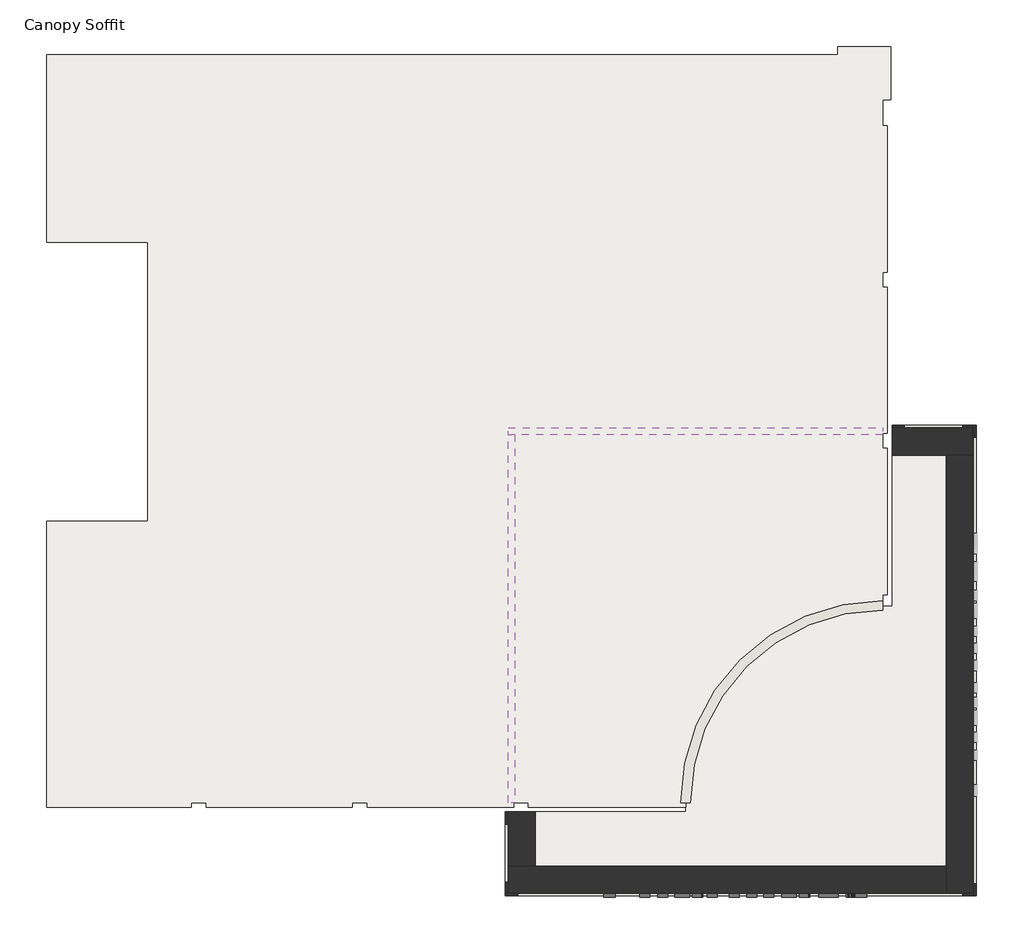
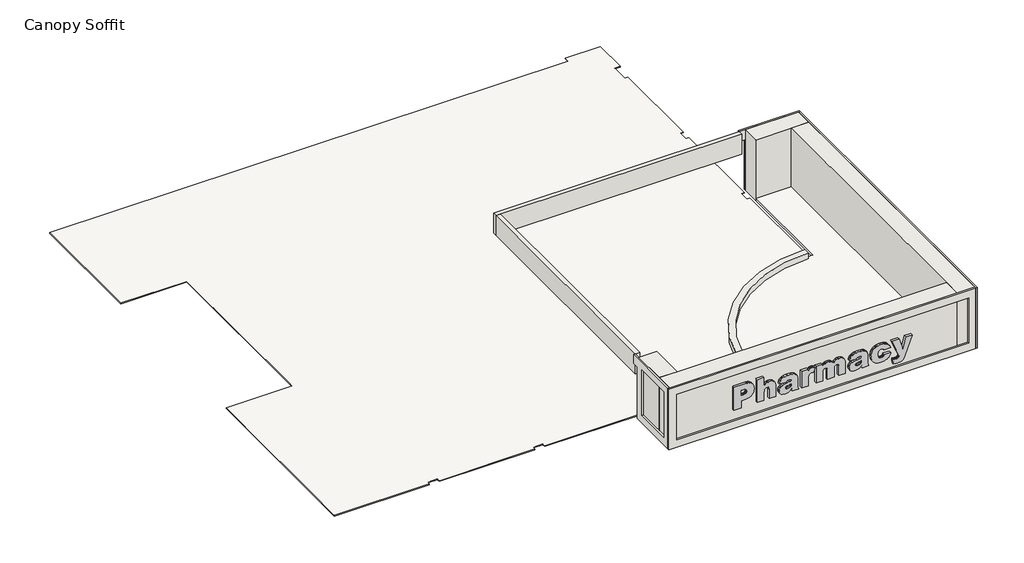
# One storey, part 1 of 2: 11 walls, 2 coverings, 1 proxy.
"""IFC4 building model written with IfcOpenShell, lengths in millimetres."""

from ifc_helpers import new_model, si_unit, point, frame, frame_2d, origin, place, context, project, spatial, polyline, circle_curve, trimmed, segment, composite_curve, outline, extrude, faceted_brep, element, save
from ifc_brep_helpers import plane_surface, cylinder_surface, revolved_surface, advanced_brep

model = new_model("IFC4")

# Units and contexts
model_context = context("Model", 3, world=origin())
ifc_project = project(units=[si_unit("LENGTHUNIT", "METRE", prefix="MILLI")], contexts=[model_context])

# Site, building, storey
site = spatial("IfcSite", under=ifc_project)
building = spatial("IfcBuilding", under=site)
storey = spatial("IfcBuildingStorey", under=building, Name="Canopy Soffit", Elevation=4572.0)

# Proxy
placement = place(None, origin())
element("IfcBuildingElementProxy", 1, Name="big", ObjectType="big", at=placement, inside=storey, context=model_context, shape_type="SweptSolid", body=[
    extrude(outline(polyline([(7079.97721, 8014.3522712), (5707.3420402, 8014.3522712), (5707.3420402, 8444.9829127), (6137.9726817, 8444.9829127), (6137.9726817, 8673.3349032), (6139.9669505, 8734.3950112), (6145.9497569, 8791.4140144), (6155.9211009, 8844.3919127), (6169.8809824, 8893.3287063), (6187.8294016, 8938.2243951), (6209.7663583, 8979.078979), (6235.6918526, 9015.8924581), (6265.6058845, 9048.6648325), (6299.0682036, 9077.4946655), (6335.6385594, 9102.4805209), (6375.3169518, 9123.6223984), (6418.103381, 9140.9202983), (6463.9978469, 9154.3742204), (6513.0003495, 9163.9841647), (6565.1108887, 9169.7501313), (6620.3294647, 9171.6721202), (6673.8461771, 9169.8914057), (6724.2154273, 9164.5492623), (6771.4372154, 9155.6456899), (6815.5115414, 9143.1806886), (6856.4384053, 9127.1542583), (6894.217807, 9107.5663991), (6928.8497466, 9084.4171109), (6960.3342242, 9057.7063938), (6988.375549, 9027.4211059), (7012.6780305, 8993.5481055), (7033.2416687, 8956.0873925), (7050.0664636, 8915.0389669), (7063.1524151, 8870.4028288), (7072.4995234, 8822.1789781), (7078.1077884, 8770.3674149), (7079.97721, 8714.9681391), (7079.97721, 8014.3522712)]), holes=[polyline([(6460.9456628, 8444.9829127), (6757.0042289, 8444.9829127), (6757.0042289, 8554.7432617), (6754.2838754, 8604.471849), (6746.122815, 8645.5794127), (6732.5210476, 8678.0659528), (6713.4785732, 8701.9314693), (6690.5461248, 8719.0420984), (6665.2744353, 8731.2639763), (6637.6635045, 8738.5971031), (6607.7133327, 8741.0414787), (6576.9877943, 8738.2291326), (6549.1534529, 8729.7920943), (6524.2103085, 8715.7303637), (6502.158361, 8696.043941), (6484.1278055, 8669.392362), (6471.2488374, 8634.4351627), (6463.5214565, 8591.1723431), (6460.9456628, 8539.6039032), (6460.9456628, 8444.9829127)])]), frame((0.0, -17607.3313057, 0.0), z_axis=(0.0, 1.0, 0.0), x_axis=(0.0, 0.0, 1.0)), (0.0, 0.0, 1.0), 152.4),
    extrude(outline(polyline([(7079.97721, 9360.0730259), (5707.3420402, 9360.0730259), (5707.3420402, 9736.8748372), (6190.5398987, 9736.8748372), (6254.0148132, 9739.6477579), (6306.9237171, 9747.96652), (6349.2666104, 9761.8311235), (6381.043493, 9781.2415683), (6404.2256357, 9805.1202266), (6420.7843091, 9832.3894704), (6430.7195131, 9863.0492998), (6434.0312478, 9897.0997146), (6431.5737304, 9927.483566), (6424.2011782, 9954.2928466), (6411.9135912, 9977.5275565), (6394.7109695, 9997.1876957), (6371.5945358, 10012.8264427), (6341.5655131, 10023.9969763), (6304.6239014, 10030.6992965), (6260.7697006, 10032.9334032), (5707.3420402, 10032.9334032), (5707.3420402, 10409.7352146), (6343.1950968, 10409.7352146), (6435.2402937, 10404.1236641), (6476.4924173, 10397.1092261), (6514.5642242, 10387.2890129), (6549.4557144, 10374.6630245), (6581.1668881, 10359.2312608), (6609.6977451, 10340.993722), (6635.0482855, 10319.9504079), (6657.3236437, 10296.4692892), (6676.6289541, 10270.9183363), (6692.9642168, 10243.2975492), (6706.3294317, 10213.606928), (6716.7245989, 10181.8464726), (6724.1497183, 10148.016183), (6730.0898138, 10074.1461013), (6727.9345579, 10023.3267443), (6721.4687902, 9976.0031072), (6710.6925107, 9932.1751901), (6695.6057195, 9891.8429929), (6675.498759, 9853.2192302), (6649.6619718, 9814.5166167), (6618.095358, 9775.7351523), (6580.7989176, 9736.8748372), (7079.97721, 9736.8748372), (7079.97721, 9360.0730259)])), frame((0.0, -17607.3313057, 0.0), z_axis=(0.0, 1.0, 0.0), x_axis=(0.0, 0.0, 1.0)), (0.0, 0.0, 1.0), 152.4),
    extrude(outline(polyline([(6353.2880025, 11001.8523466), (6380.3864028, 11012.7337605), (6402.8063209, 11025.192191), (6420.5477566, 11039.2276379), (6433.61071, 11054.8401013), (6445.5697519, 11078.3113637), (6454.1119246, 11107.091915), (6459.2372283, 11141.1817552), (6460.9456628, 11180.5808844), (6459.4474972, 11210.7281833), (6454.9530001, 11235.9867311), (6447.4621717, 11256.3565276), (6436.9750119, 11271.837573), (6422.7555797, 11283.2446591), (6404.0679341, 11291.3925778), (6380.912075, 11296.2813289), (6353.2880025, 11297.9109127), (6328.5288433, 11231.0979799), (6308.9212713, 11167.7544834), (6285.5288598, 11069.8217582), (6249.4151817, 10899.2411391), (6229.6761917, 10819.628089), (6205.3638539, 10753.629948), (6176.4781682, 10701.2467163), (6143.0191345, 10662.4783938), (6104.8027678, 10634.3286491), (6061.6450827, 10614.2216886), (6013.5460791, 10602.1575123), (5960.5057572, 10598.1361202), (5903.5754612, 10603.7082452), (5851.3762147, 10620.4246202), (5803.9080178, 10648.2852452), (5761.1708704, 10687.2901202), (5742.2466723, 10710.8730879), (5725.8457006, 10737.0449911), (5711.9679553, 10765.8058297), (5700.6134364, 10797.1556037), (5685.4740779, 10867.6219581), (5680.4276251, 10948.4440542), (5683.6867926, 11011.2355949), (5693.4642949, 11070.0845943), (5709.7601322, 11124.9910524), (5732.5743044, 11175.9549693), (5755.5724618, 11211.753244), (5785.0363869, 11247.6566532), (5820.9660797, 11283.6651969), (5863.3615402, 11319.7788749), (5782.4080261, 11333.0258136), (5707.3420402, 11361.4121108), (5707.3420402, 11722.6540259), (5764.0095001, 11697.737165), (5809.53271, 11683.5440164), (5857.1586086, 11676.9205471), (5920.1341345, 11674.712724), (6361.6987572, 11674.712724), (6397.4707483, 11672.9911476), (6434.1363822, 11667.8264186), (6510.1485779, 11647.1675023), (6546.8404954, 11632.1201364), (6579.1167666, 11614.5232605), (6606.9773916, 11594.3768746), (6630.4223704, 11571.6809787), (6658.309279, 11535.4884498), (6680.9920331, 11495.0379763), (6698.4706328, 11450.3295583), (6710.7450779, 11401.3631957), (6719.2083999, 11346.1150506), (6725.2536298, 11282.5612853), (6730.0898138, 11130.5368938), (6725.5164659, 11029.1347322), (6711.7964223, 10935.1971155), (6689.8758928, 10854.7167063), (6676.1952746, 10821.7702031), (6660.7010874, 10793.6861674), (6636.559593, 10759.8328796), (6610.3942607, 10730.1849693), (6582.2050906, 10704.7424363), (6551.9920827, 10683.5052806), (6517.8365334, 10665.5010088), (6477.8197395, 10649.7571273), (6431.9417009, 10636.2736361), (6380.2024176, 10625.0505353), (6353.2880025, 11001.8523466)]), holes=[polyline([(6164.8870968, 11297.9109127), (6118.6279459, 11297.9109127), (6069.477598, 11292.4964893), (6048.7266891, 11285.7284601), (6030.5252902, 11276.2532193), (6014.2425947, 11263.5582364), (5999.2477961, 11247.1309811), (5973.1218893, 11203.0796532), (5955.4593044, 11149.4085247), (5949.5717761, 11091.4268844), (5954.9861994, 11041.1200577), (5961.7542286, 11021.1313735), (5971.2294695, 11004.5858419), (5982.8599662, 10991.6148811), (5996.0937631, 10982.3499091), (6010.9308601, 10976.7909259), (6027.3712572, 10974.9379315), (6041.9060927, 10976.8040677), (6055.6524199, 10982.4024763), (6068.6102389, 10991.7331574), (6080.7795496, 11004.7961108), (6092.1866357, 11024.5088171), (6103.6988562, 11054.2092947), (6127.0387006, 11143.5735636), (6144.7012855, 11222.3192546), (6164.8870968, 11297.9109127)])]), frame((0.0, -17607.3313057, 0.0), z_axis=(0.0, 1.0, 0.0), x_axis=(0.0, 0.0, 1.0)), (0.0, 0.0, 1.0), 152.4),
    extrude(outline(polyline([(6703.1753987, 11890.0280447), (5707.3420402, 11890.0280447), (5707.3420402, 12266.8298561), (6043.3516912, 12266.8298561), (6154.0845337, 12270.5621285), (6245.7354765, 12281.7589457), (6318.3045196, 12300.4203077), (6347.4333287, 12312.550193), (6371.7916628, 12326.5462146), (6399.0214812, 12349.4918048), (6418.4713515, 12376.6953396), (6430.1412737, 12408.1568189), (6434.0312478, 12443.8762429), (6426.9872407, 12490.5559315), (6405.8552195, 12551.5339032), (6673.7377572, 12670.5460825), (6698.391782, 12621.0803313), (6716.0017996, 12573.6121344), (6726.5678103, 12528.1414917), (6730.0898138, 12484.6684032), (6727.5797292, 12445.7029536), (6720.0494753, 12409.9703879), (6707.4990523, 12377.470706), (6689.92846, 12348.2039079), (6665.6818312, 12320.7769625), (6633.1032985, 12293.7968384), (6592.1928618, 12267.2635356), (6542.9505213, 12241.1770542), (6703.1753987, 12241.1770542), (6703.1753987, 11890.0280447)])), frame((0.0, -17607.3313057, 0.0), z_axis=(0.0, 1.0, 0.0), x_axis=(0.0, 0.0, 1.0)), (0.0, 0.0, 1.0), 152.4),
    extrude(outline(polyline([(6703.1753987, 12724.3749127), (5707.3420402, 12724.3749127), (5707.3420402, 13101.176724), (6219.5570025, 13101.176724), (6272.7287424, 13103.8050848), (6317.8576982, 13111.6901674), (6354.9438698, 13124.8319716), (6383.9872572, 13143.2304976), (6405.8815031, 13165.7292664), (6421.5202501, 13191.1717995), (6430.9034983, 13219.5580966), (6434.0312478, 13250.8881579), (6428.2488539, 13288.3160164), (6410.9016723, 13320.6974221), (6384.0923916, 13346.1399551), (6349.9237006, 13362.7511957), (6315.7550095, 13368.4284551), (6260.3491628, 13370.3208749), (5707.3420402, 13370.3208749), (5707.3420402, 13747.1226863), (6226.706144, 13747.1226863), (6277.4335084, 13749.6721963), (6320.6963279, 13757.3207263), (6356.4946027, 13770.0682765), (6384.8283327, 13787.9148466), (6406.354608, 13809.9405105), (6421.730519, 13835.2253419), (6430.9560656, 13863.7693407), (6434.0312478, 13895.572507), (6430.7720803, 13922.7760418), (6420.9945779, 13947.6140518), (6404.6987407, 13970.0865371), (6381.8845685, 13990.1934976), (6363.0917884, 14001.6005837), (6339.9359294, 14009.7485023), (6312.4169913, 14014.6372535), (6280.5349742, 14016.2668372), (5707.3420402, 14016.2668372), (5707.3420402, 14393.0686485), (6335.6254176, 14393.0686485), (6430.4698188, 14387.5096653), (6472.8554229, 14380.5609363), (6511.8832961, 14370.8327157), (6547.5534383, 14358.3250035), (6579.8658495, 14343.0377998), (6608.8205297, 14324.9711044), (6634.4174789, 14304.1249174), (6656.8406824, 14280.8080712), (6676.2741254, 14255.3293982), (6692.717808, 14227.6888984), (6706.1717301, 14197.8865719), (6716.6358917, 14165.9224185), (6724.1102929, 14131.7964383), (6730.0898138, 14057.0589976), (6727.8951325, 14005.5694085), (6721.3110886, 13958.3377641), (6710.337682, 13915.3640642), (6694.9749128, 13876.6483089), (6673.5406301, 13839.0890324), (6644.3526829, 13799.5847688), (6607.4110712, 13758.1355182), (6562.7157949, 13714.7412806), (6601.7732371, 13691.3225854), (6635.6790921, 13664.8024245), (6664.4333598, 13635.1807977), (6688.0360402, 13602.4577051), (6706.4345662, 13565.1086975), (6719.5763704, 13521.6093254), (6727.4614529, 13471.959589), (6730.0898138, 13416.1594881), (6727.6980054, 13363.3031515), (6720.5225803, 13314.4944905), (6708.5635384, 13269.7335052), (6691.8208798, 13229.0201957), (6669.4009618, 13190.4095748), (6640.4101416, 13151.9566556), (6604.8484193, 13113.661438), (6562.7157949, 13075.5239221), (6703.1753987, 13075.5239221), (6703.1753987, 12724.3749127)])), frame((0.0, -17607.3313057, 0.0), z_axis=(0.0, 1.0, 0.0), x_axis=(0.0, 0.0, 1.0)), (0.0, 0.0, 1.0), 152.4),
    extrude(outline(polyline([(6353.2880025, 15012.1001957), (6380.3864028, 15022.9816096), (6402.8063209, 15035.44004), (6420.5477566, 15049.475487), (6433.61071, 15065.0879504), (6445.5697519, 15088.5592128), (6454.1119246, 15117.3397641), (6459.2372283, 15151.4296043), (6460.9456628, 15190.8287334), (6459.4474972, 15220.9760324), (6454.9530001, 15246.2345801), (6447.4621717, 15266.6043767), (6436.9750119, 15282.0854221), (6422.7555797, 15293.4925082), (6404.0679341, 15301.6404268), (6380.912075, 15306.529178), (6353.2880025, 15308.1587617), (6328.5288433, 15241.3458289), (6308.9212713, 15178.0023325), (6285.5288598, 15080.0696072), (6249.4151817, 14909.4889881), (6229.6761917, 14829.875938), (6205.3638539, 14763.8777971), (6176.4781682, 14711.4945654), (6143.0191345, 14672.7262429), (6104.8027678, 14644.5764982), (6061.6450827, 14624.4695377), (6013.5460791, 14612.4053614), (5960.5057572, 14608.3839693), (5903.5754612, 14613.9560943), (5851.3762147, 14630.6724693), (5803.9080178, 14658.5330943), (5761.1708704, 14697.5379693), (5742.2466723, 14721.120937), (5725.8457006, 14747.2928401), (5711.9679553, 14776.0536787), (5700.6134364, 14807.4034528), (5685.4740779, 14877.8698071), (5680.4276251, 14958.6919032), (5683.6867926, 15021.4834439), (5693.4642949, 15080.3324433), (5709.7601322, 15135.2389015), (5732.5743044, 15186.2028183), (5755.5724618, 15222.0010931), (5785.0363869, 15257.9045023), (5820.9660797, 15293.9130459), (5863.3615402, 15330.026724), (5782.4080261, 15343.2736627), (5707.3420402, 15371.6599598), (5707.3420402, 15732.9018749), (5764.0095001, 15707.9850141), (5809.53271, 15693.7918655), (5857.1586086, 15687.1683962), (5920.1341345, 15684.960573), (6361.6987572, 15684.960573), (6397.4707483, 15683.2389967), (6434.1363822, 15678.0742676), (6510.1485779, 15657.4153513), (6546.8404954, 15642.3679855), (6579.1167666, 15624.7711096), (6606.9773916, 15604.6247237), (6630.4223704, 15581.9288278), (6658.309279, 15545.7362989), (6680.9920331, 15505.2858254), (6698.4706328, 15460.5774074), (6710.7450779, 15411.6110447), (6719.2083999, 15356.3628997), (6725.2536298, 15292.8091344), (6730.0898138, 15140.7847429), (6725.5164659, 15039.3825813), (6711.7964223, 14945.4449646), (6689.8758928, 14864.9645554), (6676.1952746, 14832.0180521), (6660.7010874, 14803.9340164), (6636.559593, 14770.0807287), (6610.3942607, 14740.4328183), (6582.2050906, 14714.9902853), (6551.9920827, 14693.7531296), (6517.8365334, 14675.7488578), (6477.8197395, 14660.0049763), (6431.9417009, 14646.5214852), (6380.2024176, 14635.2983844), (6353.2880025, 15012.1001957)]), holes=[polyline([(6164.8870968, 15308.1587617), (6118.6279459, 15308.1587617), (6069.477598, 15302.7443384), (6048.7266891, 15295.9763092), (6030.5252902, 15286.5010683), (6014.2425947, 15273.8060854), (5999.2477961, 15257.3788301), (5973.1218893, 15213.3275023), (5955.4593044, 15159.6563738), (5949.5717761, 15101.6747334), (5954.9861994, 15051.3679068), (5961.7542286, 15031.3792225), (5971.2294695, 15014.833691), (5982.8599662, 15001.8627302), (5996.0937631, 14992.5977582), (6010.9308601, 14987.038775), (6027.3712572, 14985.1857806), (6041.9060927, 14987.0519168), (6055.6524199, 14992.6503254), (6068.6102389, 15001.9810064), (6080.7795496, 15015.0439598), (6092.1866357, 15034.7566662), (6103.6988562, 15064.4571438), (6127.0387006, 15153.8214127), (6144.7012855, 15232.5671037), (6164.8870968, 15308.1587617)])]), frame((0.0, -17607.3313057, 0.0), z_axis=(0.0, 1.0, 0.0), x_axis=(0.0, 0.0, 1.0)), (0.0, 0.0, 1.0), 152.4),
    extrude(outline(polyline([(6084.1438515, 16626.9651013), (6052.090991, 16613.9021479), (6024.4800603, 16597.8428631), (6001.3110594, 16578.787247), (5982.5839883, 16556.7352995), (5968.1411455, 16531.792155), (5957.8248291, 16504.062948), (5951.6350393, 16473.5476786), (5949.5717761, 16440.2463466), (5953.4617501, 16400.6500904), (5965.1316723, 16364.7072558), (5984.5815426, 16332.4178428), (6011.811361, 16303.7818513), (6046.5320078, 16280.3237308), (6088.4543633, 16263.5679304), (6137.5784276, 16253.5144501), (6193.9042006, 16250.16329), (6256.9191519, 16253.4224575), (6311.3919305, 16263.1999598), (6357.3225364, 16279.4957971), (6394.7109695, 16302.3099693), (6423.6886478, 16330.4071467), (6444.3869895, 16362.5519999), (6456.8059945, 16398.7445288), (6460.9456628, 16438.9847334), (6459.2503701, 16470.7090489), (6454.1644919, 16499.0164952), (6445.6880281, 16523.9070725), (6433.8209789, 16545.3807806), (6418.6159114, 16563.6216049), (6400.1253928, 16578.8135306), (6378.3494232, 16590.9565577), (6353.2880025, 16600.0506863), (6380.2024176, 16976.8524976), (6460.8405284, 16946.9811765), (6497.2958934, 16928.5662233), (6531.1754647, 16907.8317417), (6562.4792424, 16884.7777316), (6591.2072265, 16859.404193), (6617.359417, 16831.711126), (6640.9358138, 16801.6985306), (6661.8312825, 16768.7618837), (6679.9406888, 16732.2966624), (6695.2640325, 16692.3028666), (6707.8013138, 16648.7804964), (6717.5525325, 16601.7295517), (6724.5176888, 16551.1500327), (6730.0898138, 16439.4052712), (6727.1986169, 16358.1100701), (6718.5250261, 16284.5422499), (6704.0690414, 16218.7018107), (6683.8306628, 16160.5887523), (6667.2062805, 16126.5383375), (6646.7707749, 16092.934744), (6622.524146, 16059.7779719), (6594.466394, 16027.0680212), (6563.517445, 15996.3030574), (6530.5972253, 15968.9812464), (6495.7057351, 15945.1025881), (6458.8429742, 15924.6670825), (6404.0942177, 15902.2208808), (6342.8796935, 15886.1878796), (6275.1994016, 15876.5680789), (6201.0533421, 15873.3614787), (6130.4949951, 15876.0029814), (6067.2697749, 15883.9274893), (6011.3776814, 15897.1350026), (5962.8187147, 15915.6255212), (5919.3850517, 15938.7813802), (5878.8688692, 15965.984915), (5841.2701673, 15997.2361255), (5806.5889459, 16032.5350117), (5775.6531387, 16071.658163), (5749.2906794, 16114.3821686), (5727.5015679, 16160.7070285), (5710.2858044, 16210.6327429), (5697.2228509, 16265.6180518), (5687.8921699, 16327.1216957), (5682.2937613, 16395.1436745), (5680.4276251, 16469.6839881), (5683.3451057, 16546.6818192), (5692.0975473, 16616.6093596), (5706.68495, 16679.4666093), (5727.1073138, 16735.2535683), (5752.7863993, 16785.1792827), (5783.1439671, 16830.4527983), (5818.1800172, 16871.0741152), (5857.8945496, 16907.0432334), (5901.8933103, 16938.3207275), (5949.7820449, 16964.8671721), (6001.5607537, 16986.6825671), (6057.2294364, 17003.7669127), (6084.1438515, 16626.9651013)])), frame((0.0, -17607.3313057, 0.0), z_axis=(0.0, 1.0, 0.0), x_axis=(0.0, 0.0, 1.0)), (0.0, 0.0, 1.0), 152.4),
    extrude(outline(polyline([(6703.1753987, 17057.5957429), (5698.5107478, 17473.9281013), (5665.8796478, 17458.6310412), (5638.6366876, 17441.7569646), (5616.7818672, 17423.3058714), (5600.3151864, 17403.2777617), (5588.2641519, 17380.8578437), (5579.6562702, 17355.2313254), (5574.4915411, 17326.3982069), (5572.7699647, 17294.3584881), (5574.3206976, 17245.2344239), (5578.9728963, 17198.3707499), (5586.7265608, 17153.7674663), (5597.5816912, 17111.424573), (5326.7553893, 17141.2827523), (5309.4082077, 17289.8377075), (5303.6258138, 17394.0259315), (5309.1979388, 17488.3052352), (5316.163095, 17530.615274), (5325.9143138, 17569.7055707), (5338.451595, 17605.5761254), (5353.7749388, 17638.226938), (5371.884345, 17667.6580086), (5392.7798138, 17693.8693372), (5431.837256, 17728.589984), (5485.5083845, 17762.9426603), (5553.7931994, 17796.9273661), (5636.6917006, 17830.5441013), (6703.1753987, 18214.9155919), (6703.1753987, 17844.4218466), (6040.407927, 17663.1700825), (6703.1753987, 17463.8351957), (6703.1753987, 17057.5957429)])), frame((0.0, -17607.3313057, 0.0), z_axis=(0.0, 1.0, 0.0), x_axis=(0.0, 0.0, 1.0)), (0.0, 0.0, 1.0), 152.4),
])

# Coverings
element("IfcCovering", 2, ObjectType="24\" x 24\" ACT.", at=placement, inside=storey, context=model_context, shape_type="SweptSolid", body=[
    extrude(outline(composite_curve([segment(polyline([(18477.7022279, 12310.6936943), (18477.7022279, 11321.6811943), (18653.9147279, 11321.6811943), (18653.9147279, 5835.2811943), (18477.7022279, 5835.2811943), (18477.7022279, 5276.4811943), (18653.9147279, 5276.4811943), (18653.9147279, -209.9188057), (18477.7022279, -209.9188057), (18477.7022279, -768.7188057), (18653.9147279, -768.7188057), (18653.9147279, -6255.1188057), (18477.7022279, -6255.1188057), (18477.7022279, -6661.5188057)]), True, "CONTINUOUS"), segment(trimmed(circle_curve(frame_2d((18477.7022279, -14054.5063057)), 7392.9875), [point((18477.7022279, -6661.5188057))], [point((11086.8150464, -14230.7188057))], True, "CARTESIAN"), True, "CONTINUOUS"), segment(polyline([(11086.8150464, -14230.7188057), (5191.9147279, -14230.7188057), (5191.9147279, -14054.5063057), (4633.1147279, -14054.5063057), (4633.1147279, -14230.7188057), (-853.2852721, -14230.7188057), (-853.2852721, -14054.5063057), (-1412.0852721, -14054.5063057), (-1412.0852721, -14230.7188057), (-6898.4852721, -14230.7188057), (-6898.4852721, -14054.5063057), (-7457.2852721, -14054.5063057), (-7457.2852721, -14230.7188057), (-12883.3602721, -14230.7188057), (-12883.3602721, -3500.0125557), (-9095.5852721, -3500.0125557), (-9095.5852721, 6956.8499443), (-12883.3602721, 6956.8499443), (-12883.3602721, 13993.4436943), (16794.9522279, 13993.4436943), (16794.9522279, 14298.2436943), (18782.5022279, 14298.2436943), (18782.5022279, 12310.6936943), (18477.7022279, 12310.6936943)]), True, "CONTINUOUS")], self_intersect=False)), frame((0.0, 0.0, 4572.0), z_axis=(0.0, 0.0, 1.0), x_axis=(1.0, 0.0, 0.0)), (0.0, 0.0, 1.0), 38.1),
])
element("IfcCovering", 3, ObjectType="GWB on Mtl. Stud", at=placement, inside=storey, context=model_context, shape_type="SweptSolid", body=[
    extrude(outline(composite_curve([segment(polyline([(5445.9147279, -14406.9313057), (11093.1195861, -14406.9313057)]), True, "CONTINUOUS"), segment(trimmed(circle_curve(frame_2d((18477.7022279, -14054.5063057)), 7392.9875), [point((11093.1195861, -14406.9313057))], [point((18830.1272279, -6669.9236638))], False, "CARTESIAN"), True, "CONTINUOUS"), segment(polyline([(18830.1272279, -6669.9236638), (18830.1272279, -1022.7188057), (20862.1272279, -1022.7188057), (20862.1272279, -16438.9313057), (5445.9147279, -16438.9313057), (5445.9147279, -14406.9313057)]), True, "CONTINUOUS")], self_intersect=False)), frame((0.0, 0.0, 4572.0), z_axis=(0.0, 0.0, 1.0), x_axis=(1.0, 0.0, 0.0)), (0.0, 0.0, 1.0), 107.95),
])

# Walls
element("IfcWall", 4, ObjectType="Exterior - Brick on Mtl. Stud - No Cap", at=placement, inside=storey, context=model_context, shape_type="AdvancedBrep", body=[
    advanced_brep(
    [(18477.7022279, -6485.3063057, 5029.2), (10908.5022279, -14054.5063057, 5029.2), (11260.9272279, -14054.5063057, 5029.2), (18477.7022279, -6837.7313057, 5029.2), (10908.5022279, -14054.5063057, 3048.0), (18477.7022279, -6485.3063057, 3048.0), (18477.7022279, -6837.7313057, 3048.0), (18477.7022279, -6837.7313057, 4625.5040439), (11260.9272279, -14054.5063057, 4625.5040439), (11260.9272279, -14054.5063057, 3048.0)],
    [
        (0, 1, circle_curve(frame((18477.7022279, -14054.5063057, 5029.2), z_axis=(0.0, 0.0, 1.0), x_axis=(1.0, 0.0, 0.0)), 7569.2)),
        (1, 2),
        (2, 3, circle_curve(frame((18477.7022279, -14054.5063057, 5029.2), z_axis=(0.0, 0.0, -1.0), x_axis=(1.0, 0.0, 0.0)), 7216.775)),
        (3, 0),
        (4, 1),
        (0, 5),
        (5, 4, circle_curve(frame((18477.7022279, -14054.5063057, 3048.0), z_axis=(0.0, 0.0, 1.0), x_axis=(1.0, 0.0, 0.0)), 7569.2)),
        (6, 7),
        (7, 3),
        (2, 8),
        (8, 9),
        (9, 6, circle_curve(frame((18477.7022279, -14054.5063057, 3048.0), z_axis=(0.0, 0.0, -1.0), x_axis=(1.0, 0.0, 0.0)), 7216.775)),
        (6, 5),
        (4, 9),
    ],
    [
        plane_surface(frame((26046.9022279, -14054.5063057, 5029.2), z_axis=(0.0, 0.0, 1.0), x_axis=(0.0, 1.0, 0.0))),
        cylinder_surface(frame((18477.7022279, -14054.5063057, 4572.0), z_axis=(0.0, 0.0, 1.0), x_axis=(1.0, 0.0, 0.0)), 7569.2),
        revolved_surface(polyline([(25694.477227900003, -14054.5063057, 3048.0), (25694.477227900003, -14054.5063057, 5029.2)]), (18477.7022279, -14054.5063057, 4572.0), (0.0, 0.0, -1.0)),
        plane_surface(frame((18477.7022279, 12134.4811943, 7620.0), z_axis=(1.0, 0.0, 0.0), x_axis=(0.0, 0.0, -1.0))),
        plane_surface(frame((-12953.2102721, -14054.5063057, 7620.0), z_axis=(0.0, -1.0, 0.0), x_axis=(1.0, 0.0, 0.0))),
        plane_surface(frame((25883.3897279, -14054.5063057, 3048.0), z_axis=(0.0, 0.0, -1.0), x_axis=(0.0, 1.0, 0.0))),
    ],
    [
        (0, [[1, 2, 3, 4]]),
        (1, [[5, -1, 6, 7]]),
        (2, [[8, 9, -3, 10, 11, 12]]),
        (3, [[-4, -9, -8, 13, -6]]),
        (4, [[-2, -5, 14, -11, -10]]),
        (5, [[-13, -12, -14, -7]]),
    ],
),
])
element("IfcWall", 5, ObjectType="Exterior - EIFS Canopy Roof Wall", at=placement, inside=storey, context=model_context, shape_type="Brep", body=[
    faceted_brep([(18477.7022279, -6.7188057, 7016.75), (4429.9147279, -6.7188057, 7016.75), (4429.9147279, -6.7188057, 8229.6), (18477.7022279, -6.7188057, 8229.6), (18477.7022279, -254.3688057, 7016.75), (18477.7022279, -254.3688057, 8229.6), (4677.5647279, -254.3688057, 8229.6), (4429.9147279, -254.3688057, 8229.6), (4429.9147279, -254.3688057, 7016.75), (4677.5647279, -254.3688057, 7016.75)], [[[0, 1, 2, 3]], [[4, 5, 6, 7, 8, 9]], [[3, 2, 7, 6, 5]], [[0, 3, 5, 4]], [[2, 1, 8, 7]], [[1, 0, 4, 9, 8]]]),
])
element("IfcWall", 6, ObjectType="Exterior - EIFS Canopy Roof Wall", at=placement, inside=storey, context=model_context, shape_type="SweptSolid", body=[
    extrude(outline(polyline([(4677.5647279, -254.3688057), (4677.5647279, -14054.5063057), (4429.9147279, -14054.5063057), (4429.9147279, -254.3688057), (4677.5647279, -254.3688057)])), frame((0.0, 0.0, 7016.75), z_axis=(0.0, 0.0, 1.0), x_axis=(1.0, 0.0, 0.0)), (0.0, 0.0, 1.0), 1212.85),
])
element("IfcWall", 7, ObjectType="Exterior - EIFS Canopy Wall", at=placement, inside=storey, context=model_context, shape_type="Brep", body=[
    faceted_brep([(18830.1272279, -1022.7188057, 4572.0), (20862.1272279, -1022.7188057, 4572.0), (21878.1272279, -1022.7188057, 4572.0), (21878.1272279, -1022.7188057, 8229.6), (20862.1272279, -1022.7188057, 8229.6), (18830.1272279, -1022.7188057, 8229.6), (18830.1272279, -6.7188057, 4572.0), (18830.1272279, -6.7188057, 7620.0), (18830.1272279, -6.7188057, 8229.6), (21878.1272279, -6.7188057, 8229.6), (21878.1272279, -6.7188057, 4572.0)], [[[0, 1, 2, 3, 4, 5]], [[6, 7, 8, 9, 10]], [[2, 1, 0, 6, 10]], [[5, 4, 3, 9, 8]], [[0, 5, 8, 7, 6]], [[3, 2, 10, 9]]]),
])
element("IfcWall", 8, ObjectType="Exterior - EIFS Canopy Wall", at=placement, inside=storey, context=model_context, shape_type="Brep", body=[
    faceted_brep([(20862.1272279, -1022.7188057, 4572.0), (20862.1272279, -16438.9313057, 4572.0), (20862.1272279, -17454.9313057, 4572.0), (20862.1272279, -17454.9313057, 8229.6), (20862.1272279, -16438.9313057, 8229.6), (20862.1272279, -1022.7188057, 8229.6), (21878.1272279, -1022.7188057, 4572.0), (21878.1272279, -1022.7188057, 8229.6), (21878.1272279, -17454.9313057, 8229.6), (21878.1272279, -17454.9313057, 4572.0)], [[[0, 1, 2, 3, 4, 5]], [[6, 7, 8, 9]], [[2, 1, 0, 6, 9]], [[5, 4, 3, 8, 7]], [[0, 5, 7, 6]], [[3, 2, 9, 8]]]),
])
element("IfcWall", 9, ObjectType="Exterior - EIFS Canopy Wall", at=placement, inside=storey, context=model_context, shape_type="Brep", body=[
    faceted_brep([(20862.1272279, -16438.9313057, 4572.0), (5445.9147279, -16438.9313057, 4572.0), (4429.9147279, -16438.9313057, 4572.0), (4429.9147279, -16438.9313057, 8229.6), (5445.9147279, -16438.9313057, 8229.6), (20862.1272279, -16438.9313057, 8229.6), (20862.1272279, -17454.9313057, 4572.0), (20862.1272279, -17454.9313057, 8229.6), (4429.9147279, -17454.9313057, 8229.6), (4429.9147279, -17454.9313057, 4572.0)], [[[0, 1, 2, 3, 4, 5]], [[6, 7, 8, 9]], [[2, 1, 0, 6, 9]], [[5, 4, 3, 8, 7]], [[0, 5, 7, 6]], [[3, 2, 9, 8]]]),
])
element("IfcWall", 10, ObjectType="Exterior - EIFS Canopy Wall", at=placement, inside=storey, context=model_context, shape_type="Brep", body=[
    faceted_brep([(5445.9147279, -16438.9313057, 4572.0), (5445.9147279, -14406.9313057, 4572.0), (5445.9147279, -14406.9313057, 8229.6), (5445.9147279, -16438.9313057, 8229.6), (4429.9147279, -16438.9313057, 4572.0), (4429.9147279, -16438.9313057, 8229.6), (4429.9147279, -14406.9313057, 8229.6), (4429.9147279, -14406.9313057, 7683.5), (4429.9147279, -14406.9313057, 4572.0)], [[[0, 1, 2, 3]], [[4, 5, 6, 7, 8]], [[1, 0, 4, 8]], [[2, 1, 8, 7, 6]], [[3, 2, 6, 5]], [[0, 3, 5, 4]]]),
])
element("IfcWall", 11, ObjectType="Exterior - EIFS Details", at=placement, inside=storey, context=model_context, shape_type="Brep", body=[
    faceted_brep([(18830.1272279, -6.7188057, 4572.0), (21878.1272279, -6.7188057, 4572.0), (21979.7272279, -6.7188057, 4572.0), (21979.7272279, -6.7188057, 8229.6), (21878.1272279, -6.7188057, 8229.6), (18830.1272279, -6.7188057, 8229.6), (18477.7022279, -6.7188057, 8229.6), (18477.7022279, -6.7188057, 7620.0), (18830.1272279, -6.7188057, 7620.0), (21471.7272279, -6.7188057, 5029.2), (19287.3272279, -6.7188057, 5029.2), (19287.3272279, -6.7188057, 7772.4), (21471.7272279, -6.7188057, 7772.4), (18830.1272279, 94.8811943, 4572.0), (18830.1272279, 94.8811943, 7620.0), (18477.7022279, 94.8811943, 7620.0), (18477.7022279, 94.8811943, 8229.6), (21979.7272279, 94.8811943, 8229.6), (21979.7272279, 94.8811943, 4572.0), (21471.7272279, 94.8811943, 5029.2), (21471.7272279, 94.8811943, 7772.4), (19287.3272279, 94.8811943, 7772.4), (19287.3272279, 94.8811943, 5029.2)], [[[0, 1, 2, 3, 4, 5, 6, 7, 8], [9, 10, 11, 12]], [[13, 14, 15, 16, 17, 18], [19, 20, 21, 22]], [[3, 2, 18, 17]], [[2, 1, 0, 13, 18]], [[6, 5, 4, 3, 17, 16]], [[0, 8, 14, 13]], [[10, 9, 19, 22]], [[11, 10, 22, 21]], [[12, 11, 21, 20]], [[9, 12, 20, 19]], [[7, 6, 16, 15]], [[8, 7, 15, 14]]]),
])
element("IfcWall", 12, ObjectType="Exterior - EIFS Details", at=placement, inside=storey, context=model_context, shape_type="Brep", body=[
    faceted_brep([(21878.1272279, -6.7188057, 4572.0), (21878.1272279, -1022.7188057, 4572.0), (21878.1272279, -17454.9313057, 4572.0), (21878.1272279, -17556.5313057, 4572.0), (21878.1272279, -17556.5313057, 8229.6), (21878.1272279, -17454.9313057, 8229.6), (21878.1272279, -1022.7188057, 8229.6), (21878.1272279, -6.7188057, 8229.6), (21878.1272279, -362.3188057, 5029.2), (21878.1272279, -362.3188057, 7772.4), (21878.1272279, -17099.3313057, 7772.4), (21878.1272279, -17099.3313057, 5029.2), (21979.7272279, -6.7188057, 4572.0), (21979.7272279, -6.7188057, 8229.6), (21979.7272279, -17556.5313057, 8229.6), (21979.7272279, -17556.5313057, 4572.0), (21979.7272279, -362.3188057, 5029.2), (21979.7272279, -17099.3313057, 5029.2), (21979.7272279, -17099.3313057, 7772.4), (21979.7272279, -362.3188057, 7772.4)], [[[0, 1, 2, 3, 4, 5, 6, 7], [8, 9, 10, 11]], [[12, 13, 14, 15], [16, 17, 18, 19]], [[0, 7, 13, 12]], [[4, 3, 15, 14]], [[3, 2, 1, 0, 12, 15]], [[7, 6, 5, 4, 14, 13]], [[9, 8, 16, 19]], [[10, 9, 19, 18]], [[11, 10, 18, 17]], [[8, 11, 17, 16]]]),
])
element("IfcWall", 13, ObjectType="Exterior - EIFS Details", at=placement, inside=storey, context=model_context, shape_type="Brep", body=[
    faceted_brep([(21878.1272279, -17454.9313057, 4572.0), (20862.1272279, -17454.9313057, 4572.0), (4429.9147279, -17454.9313057, 4572.0), (4328.3147279, -17454.9313057, 4572.0), (4328.3147279, -17454.9313057, 8229.6), (4429.9147279, -17454.9313057, 8229.6), (20862.1272279, -17454.9313057, 8229.6), (21878.1272279, -17454.9313057, 8229.6), (4785.5147279, -17454.9313057, 5029.2), (21471.7272279, -17454.9313057, 5029.2), (21471.7272279, -17454.9313057, 7772.4), (4785.5147279, -17454.9313057, 7772.4), (21878.1272279, -17556.5313057, 4572.0), (21878.1272279, -17556.5313057, 8229.6), (4328.3147279, -17556.5313057, 8229.6), (4328.3147279, -17556.5313057, 4572.0), (4785.5147279, -17556.5313057, 5029.2), (4785.5147279, -17556.5313057, 7772.4), (21471.7272279, -17556.5313057, 7772.4), (21471.7272279, -17556.5313057, 5029.2)], [[[0, 1, 2, 3, 4, 5, 6, 7], [8, 9, 10, 11]], [[12, 13, 14, 15], [16, 17, 18, 19]], [[0, 7, 13, 12]], [[4, 3, 15, 14]], [[3, 2, 1, 0, 12, 15]], [[7, 6, 5, 4, 14, 13]], [[9, 8, 16, 19]], [[10, 9, 19, 18]], [[11, 10, 18, 17]], [[8, 11, 17, 16]]]),
])
element("IfcWall", 14, ObjectType="Exterior - EIFS Details", at=placement, inside=storey, context=model_context, shape_type="Brep", body=[
    faceted_brep([(4429.9147279, -17454.9313057, 4572.0), (4429.9147279, -16438.9313057, 4572.0), (4429.9147279, -14406.9313057, 4572.0), (4429.9147279, -14406.9313057, 7683.5), (4429.9147279, -14054.5063057, 7683.5), (4429.9147279, -14054.5063057, 8229.6), (4429.9147279, -14406.9313057, 8229.6), (4429.9147279, -16438.9313057, 8229.6), (4429.9147279, -17454.9313057, 8229.6), (4429.9147279, -14864.1313057, 7772.4), (4429.9147279, -14864.1313057, 5029.2), (4429.9147279, -17048.5313057, 5029.2), (4429.9147279, -17048.5313057, 7772.4), (4328.3147279, -17454.9313057, 4572.0), (4328.3147279, -17454.9313057, 8229.6), (4328.3147279, -14054.5063057, 8229.6), (4328.3147279, -14054.5063057, 7683.5), (4328.3147279, -14406.9313057, 7683.5), (4328.3147279, -14406.9313057, 4572.0), (4328.3147279, -14864.1313057, 7772.4), (4328.3147279, -17048.5313057, 7772.4), (4328.3147279, -17048.5313057, 5029.2), (4328.3147279, -14864.1313057, 5029.2)], [[[0, 1, 2, 3, 4, 5, 6, 7, 8], [9, 10, 11, 12]], [[13, 14, 15, 16, 17, 18], [19, 20, 21, 22]], [[0, 8, 14, 13]], [[2, 1, 0, 13, 18]], [[3, 2, 18, 17]], [[8, 7, 6, 5, 15, 14]], [[10, 9, 19, 22]], [[11, 10, 22, 21]], [[12, 11, 21, 20]], [[9, 12, 20, 19]], [[4, 3, 17, 16]], [[5, 4, 16, 15]]]),
])

save(model, "model.ifc")

# Revit data of these elements
# Type "24\" x 24\" ACT."
#   Assembly Code = "C3030220"
#   built-in parameter 1002203 = 1 (stored number, unit not read)
#   built-in parameter 1002202 = 1 (stored number, unit not read)
#   Layers, outside or top first: 25.4 mm "Metal - Stud Layer" (function 1); 12.7 mm "Acoustic Ceiling Tile 24\" x 24\"" (function 5)
# Type "GWB on Mtl. Stud"
#   Assembly Code = "C3030220"
#   built-in parameter 1002203 = 1 (stored number, unit not read)
#   built-in parameter 1002202 = 1 (stored number, unit not read)
#   Layers, outside or top first: 92.075 mm "Metal - Stud Layer" (function 1); 15.875 mm "Gypsum Wall Board" (function 5)
# Type "Exterior - Brick on Mtl. Stud - No Cap"
#   Assembly Code = "B2010158"
#   Layers, outside or top first: 92.075 mm "Masonry - Brick" (function 4); 76.2 mm "Misc. Air Layers - Air Space" (function 3); 0 mm "Air Barrier - Air Infiltration Barrier" (function 100); 19.05 mm "Wood - Sheathing - plywood" (function 2); 152.4 mm "Metal - Stud Layer" (function 1); 0 mm "Vapor / Moisture Barriers - Vapor Retarder" (function 100); 12.7 mm "Gypsum Wall Board" (function 5)
# Type "Exterior - EIFS Canopy Roof Wall"
#   Assembly Code = "B2010100"
#   Layers, outside or top first: 76.2 mm "EIFS - Exterior Insulation and Finish System" (function 4); 0 mm "Air Barrier - Air Infiltration Barrier" (function 100); 19.05 mm "Wood - Sheathing - plywood" (function 2); 152.4 mm "Metal - Stud Layer" (function 1)
# Type "Exterior - EIFS Canopy Wall"
#   Assembly Code = "B2010100"
#   Layers, outside or top first: 76.2 mm "EIFS - Exterior Insulation and Finish System" (function 4); 0 mm "Air Barrier - Air Infiltration Barrier" (function 100); 19.05 mm "Wood - Sheathing - plywood" (function 2); 152.4 mm "Metal - Stud Layer" (function 1); 539.75 mm "Default Form" (function 1); 152.4 mm "Metal - Stud Layer" (function 1); 0 mm "Vapor / Moisture Barriers - Vapor Retarder" (function 100); 76.2 mm "EIFS - Exterior Insulation and Finish System" (function 5)
# Type "Exterior - EIFS Details"
#   Assembly Code = "B2010100"
#   Layers, outside or top first: 101.6 mm "EIFS - Exterior Insulation and Finish System" (function 4)
# Element 1 (IfcBuildingElementProxy, "big")
#   Phase Created = New Construction
#   Materials on its faces: "Paint - Red"
# Element 2 (IfcCovering, "24\" x 24\" ACT.")
#   Height Offset From Level = 0 mm
#   Phase Created = New Construction
#   Materials on its faces: "Acoustic Ceiling Tile 24\" x 24\"", "Metal - Stud Layer"
# Element 3 (IfcCovering, "GWB on Mtl. Stud")
#   Height Offset From Level = 0 mm
#   Phase Created = New Construction
#   Materials on its faces: "Gypsum Wall Board", "Metal - Stud Layer"
# Element 4 (IfcWall, "Exterior - Brick on Mtl. Stud - No Cap")
#   Top Offset = 457.2 mm
#   Base Offset = 0 mm
#   Unconnected Height = 1583.854 mm
#   wall height = 457.2 mm
#   Phase Created = New Construction
#   Materials on its faces: "Default Wall", "Gypsum Wall Board", "Masonry - Brick"
# Element 5 (IfcWall, "Exterior - EIFS Canopy Roof Wall")
#   Top Offset = 304.8 mm
#   Base Offset = 0 mm
#   wall height = 3657.6 mm
#   Phase Created = New Construction
#   Base Constraint = Canopy Soffit
#   Top Constraint = Upper Parapet
#   Materials on its faces: "Default Wall", "EIFS - Exterior Insulation and Finish System", "Metal - Stud Layer"
# Element 6 (IfcWall, "Exterior - EIFS Canopy Roof Wall")
#   Top Offset = 304.8 mm
#   Base Offset = 0 mm
#   wall height = 3657.6 mm
#   Phase Created = New Construction
#   Base Constraint = Canopy Soffit
#   Top Constraint = Upper Parapet
#   Materials on its faces: "Default Wall", "Metal - Stud Layer", "EIFS - Exterior Insulation and Finish System"
# Elements 7, 8, 9 (IfcWall, "Exterior - EIFS Canopy Wall")
#   Top Offset = 304.8 mm
#   Base Offset = 0 mm
#   wall height = 3657.6 mm
#   Phase Created = New Construction
#   Base Constraint = Canopy Soffit
#   Top Constraint = Upper Parapet
#   Materials on its faces: "EIFS - Exterior Insulation and Finish System", "Default Wall"
# Element 10 (IfcWall, "Exterior - EIFS Canopy Wall")
#   Top Offset = 304.8 mm
#   Base Offset = 0 mm
#   wall height = 3657.6 mm
#   Phase Created = New Construction
#   Base Constraint = Canopy Soffit
#   Top Constraint = Upper Parapet
#   Materials on its faces: "Default Wall", "EIFS - Exterior Insulation and Finish System"
# Elements 11, 12, 13, 14 (IfcWall, "Exterior - EIFS Details")
#   Top Offset = 304.8 mm
#   Base Offset = 0 mm
#   wall height = 3657.6 mm
#   Phase Created = New Construction
#   Base Constraint = Canopy Soffit
#   Top Constraint = Upper Parapet
#   Materials on its faces: "EIFS - Exterior Insulation and Finish System"
# Materials
#   "Metal - Stud Layer": class "Metal", colour RGB 199 199 199, transparency 0, Cost = 0
#   "Acoustic Ceiling Tile 24\" x 24\"": class "Miscellaneous", colour RGB 232 232 232, transparency 0, Description = "Interior finish", Cost = 0
#   "Gypsum Wall Board": class "Paint", colour RGB 127 127 127, transparency 0, Description = "Interior finish", Cost = 0
#   "Masonry - Brick": class "Brick", colour RGB 130 72 45, transparency 0, Cost = 0
#   "Misc. Air Layers - Air Space": class "Miscellaneous", colour RGB 255 255 255, transparency 0, Cost = 0
#   "Air Barrier - Air Infiltration Barrier": class "Miscellaneous", colour RGB 127 127 127, transparency 0, Cost = 0
#   "Wood - Sheathing - plywood": class "Wood", colour RGB 212 179 113, transparency 0, Cost = 0
#   "Vapor / Moisture Barriers - Vapor Retarder": class "Miscellaneous", colour RGB 127 127 127, transparency 0, Cost = 0
#   "EIFS - Exterior Insulation and Finish System": class "Stucco", colour RGB 224 218 190, transparency 0, Description = "Exterior finish", Cost = 0
#   "Default Form": class "Miscellaneous", colour RGB 185 189 196, transparency 0.9, Cost = 0
#   "Paint - Red": class "Paint", colour RGB 204 0 0, transparency 0, Cost = 0
#   "Default Wall": class "Miscellaneous", colour RGB 128 128 128, transparency 0, Cost = 0
